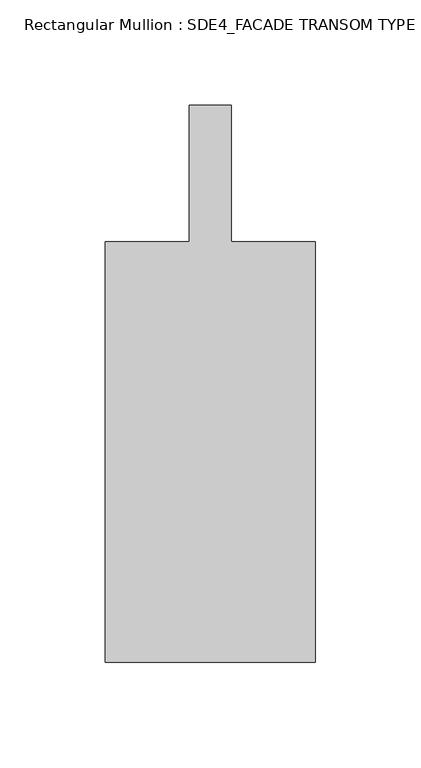
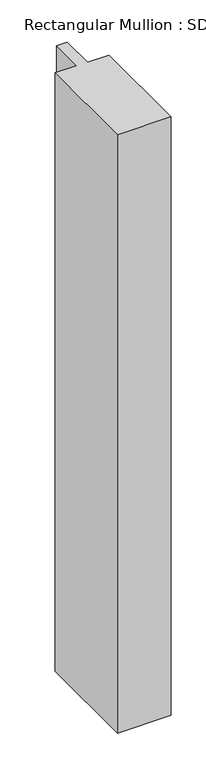
"""IFC4 building model written with IfcOpenShell, lengths in millimetres: member geometry, Rectangular Mullion : SDE4_FACADE TRANSOM TYPE 2."""

from ifc_helpers import new_model, si_unit, frame, origin, place, context, project, spatial, polyline, outline, extrude, source, transform, mapped, element, save


def rectangular_mullion_sde4_facade_transom_type_2_0249099c(model_context):
    return source(origin(), model_context, "Body", "SweptSolid", [
        extrude(outline(polyline([(50.0, -132.5), (-50.0, -132.5), (-50.0, 67.5), (-10.0, 67.5), (-10.0, 132.5), (10.0, 132.5), (10.0, 67.5), (50.0, 67.5), (50.0, -132.5)])), frame((0.0, 0.0, -1171.5000001), z_axis=(0.0, 0.0, 1.0), x_axis=(1.0, 0.0, 0.0)), (0.0, 0.0, 1.0), 1171.5000001),
    ])


if __name__ == "__main__":
    model = new_model("IFC4")
    model_context = context("Model", 3, world=origin())
    ifc_project = project(units=[si_unit("LENGTHUNIT", "METRE", prefix="MILLI")], contexts=[model_context])
    site = spatial("IfcSite", under=ifc_project)
    building = spatial("IfcBuilding", under=site)
    placement = place(None, origin())
    rectangular_mullion_sde4_facade_transom_type_2_shape = rectangular_mullion_sde4_facade_transom_type_2_0249099c(model_context)
    element("IfcMember", 1, ObjectType="Rectangular Mullion : SDE4_FACADE TRANSOM TYPE 2", at=placement, inside=building, context=model_context, shape_type="MappedRepresentation", body=[
        mapped(rectangular_mullion_sde4_facade_transom_type_2_shape, transform((0.0, 0.0, 0.0), x_axis=(1.0, 0.0, 0.0), y_axis=(0.0, 1.0, 0.0), z_axis=(0.0, 0.0, 1.0))),
    ])
    save(model, "model.ifc")

# Revit data of these elements
# Type "Rectangular Mullion : SDE4_FACADE TRANSOM TYPE 2"
#   built-in parameter 1007322 = 0.869423 (stored number, unit not read)
#   built-in parameter 1007321 = 0.164042 (stored number, unit not read)
#   built-in parameter 1007320 = 0.164042 (stored number, unit not read)
